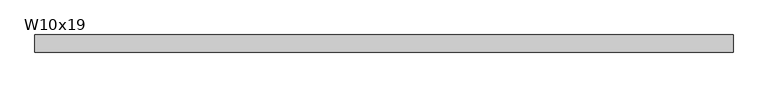
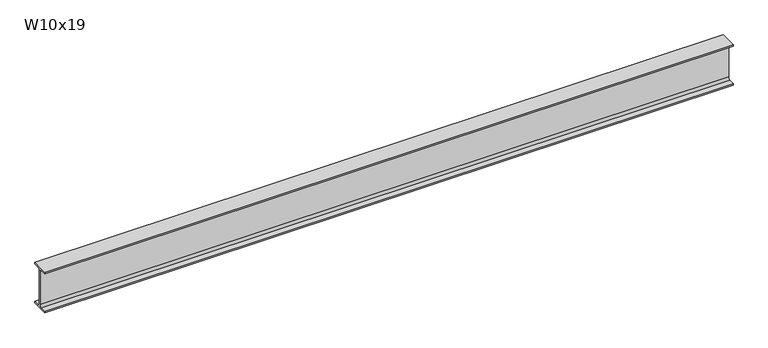
"""IFC4 building model written with IfcOpenShell, lengths in millimetres: beam geometry, RME W-Wide Flange : W10x19."""

from ifc_helpers import new_model, si_unit, point, frame, frame_2d, origin, place, context, project, spatial, polyline, circle_curve, trimmed, segment, composite_curve, outline, extrude, source, transform, mapped, element, save


def w10x19_618fdea2(model_context):
    return source(origin(), model_context, "Body", "SweptSolid", [
        extrude(outline(composite_curve([segment(polyline([(51.054, -119.507), (51.054, -129.54), (-51.054, -129.54), (-51.054, -119.507), (-16.9545, -119.507)]), True, "CONTINUOUS"), segment(trimmed(circle_curve(frame_2d((-16.9545, -105.7275)), 13.7795), [point((-16.9545, -119.507))], [point((-3.175, -105.7275))], True, "CARTESIAN"), True, "CONTINUOUS"), segment(polyline([(-3.175, -105.7275), (-3.175, 105.7275)]), True, "CONTINUOUS"), segment(trimmed(circle_curve(frame_2d((-16.9545, 105.7275)), 13.7795), [point((-3.175, 105.7275))], [point((-16.9545, 119.507))], True, "CARTESIAN"), True, "CONTINUOUS"), segment(polyline([(-16.9545, 119.507), (-51.054, 119.507), (-51.054, 129.54), (51.054, 129.54), (51.054, 119.507), (16.9545, 119.507)]), True, "CONTINUOUS"), segment(trimmed(circle_curve(frame_2d((16.9545, 105.7275)), 13.7795), [point((16.9545, 119.507))], [point((3.175, 105.7275))], True, "CARTESIAN"), True, "CONTINUOUS"), segment(polyline([(3.175, 105.7275), (3.175, -105.7275)]), True, "CONTINUOUS"), segment(trimmed(circle_curve(frame_2d((16.9545, -105.7275)), 13.7795), [point((3.175, -105.7275))], [point((16.9545, -119.507))], True, "CARTESIAN"), True, "CONTINUOUS"), segment(polyline([(16.9545, -119.507), (51.054, -119.507)]), True, "CONTINUOUS")], self_intersect=False)), frame((-2085.0946126, 0.0, 0.0), z_axis=(1.0, 0.0, 0.0), x_axis=(0.0, 1.0, 0.0)), (0.0, 0.0, 1.0), 4157.4892245),
    ])


if __name__ == "__main__":
    model = new_model("IFC4")
    model_context = context("Model", 3, world=origin())
    ifc_project = project(units=[si_unit("LENGTHUNIT", "METRE", prefix="MILLI")], contexts=[model_context])
    site = spatial("IfcSite", under=ifc_project)
    building = spatial("IfcBuilding", under=site)
    placement = place(None, origin())
    w10x19_shape = w10x19_618fdea2(model_context)
    element("IfcBeam", 1, ObjectType="RME W-Wide Flange : W10x19", at=placement, inside=building, context=model_context, shape_type="MappedRepresentation", body=[
        mapped(w10x19_shape, transform((0.0, 0.0, 0.0), x_axis=(1.0, 0.0, 0.0), y_axis=(0.0, 1.0, 0.0), z_axis=(0.0, 0.0, 1.0))),
    ])
    save(model, "model.ifc")

# Revit data of these elements
# Type "RME W-Wide Flange : W10x19"
#   WELD P [instance default] = ""
#   WELD LE [instance default] = ""
#   WELD D [instance default] = ""
#   TOP SECTION SIZE [instance default] = ""
#   TOP SECTION LENGTH [instance default] = ""
#   REMARKS [instance default] = ""
#   REINF TYPE [instance default] = ""
#   Nominal Size = "W24"
#   End Bearing Capacity [instance default] = ""
#   BOT SECTION SIZE [instance default] = ""
#   BOT SECTION LENGTH [instance default] = ""
#   Assembly Code = "B10"
#   W = 19
#   Start Extension Calculation [instance default] = 10' - 0"
#   Start Extension [instance default] = -0' - 0 1/2"
#   End Extension Calculation [instance default] = 10' - 0"
#   End Extension [instance default] = -0' - 0 1/2"
#   Length [instance default] = 5' - 0"
#   bf = 0' - 4.02"
#   d = 0' - 10.2"
#   k = 0' - 0 15/16"
#   k2 = 0' - 0.5425"
#   tf = 0' - 0.395"
#   tw = 0' - 0 1/4"
#   A = 0.0390278 SF
#   Structural Material [instance default] = Metal - Steel - ASTM A992
# Element 1 (IfcBeam, "RME W-Wide Flange : W10x19")
#   Length = 13' - 8.18068"
#   Materials on its faces: "Metal - Steel - ASTM A992"
# Materials
#   "Metal - Steel - ASTM A992": class "Metal", colour RGB 255 128 0, transparency 0
